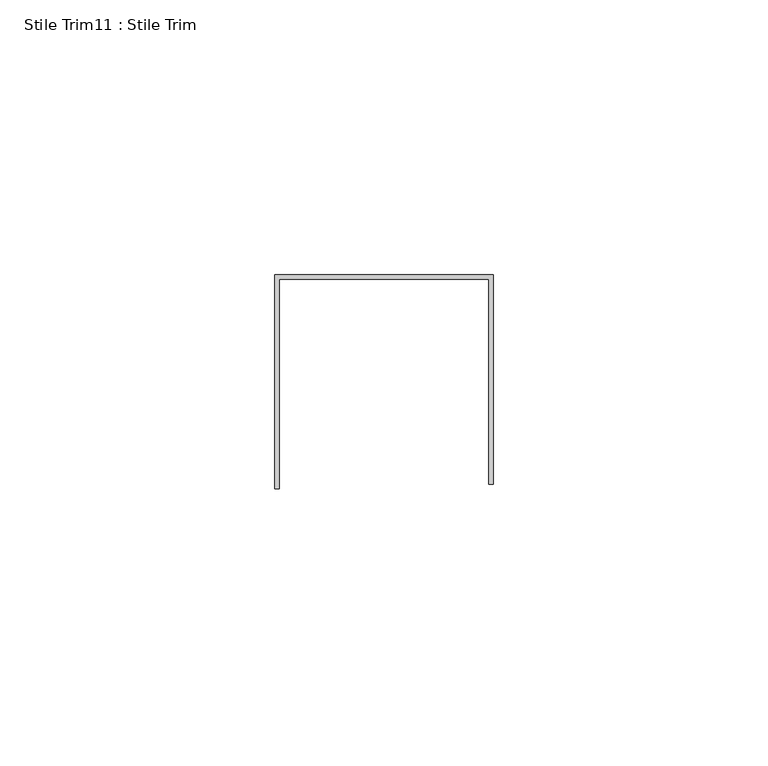
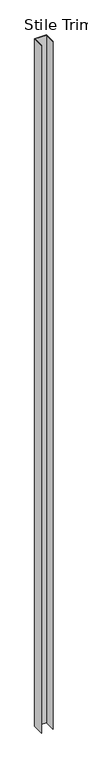
"""IFC4 building model written with IfcOpenShell, lengths in millimetres: proxy geometry, Stile Trim11 : Stile Trim."""

from ifc_helpers import new_model, si_unit, frame, origin, place, context, project, spatial, polyline, outline, extrude, source, transform, mapped, element, save


def stile_trim11_stile_trim_282884a6(model_context):
    return source(origin(), model_context, "Body", "SweptSolid", [
        extrude(outline(polyline([(587327.0060739, -536293.7663841), (587366.6808739, -536293.7663841), (587366.6808739, -536331.8663841), (587365.8934739, -536331.8663841), (587365.8934739, -536294.5537841), (587327.7934739, -536294.5537841), (587327.7934739, -536332.6537841), (587327.0060739, -536332.6537841), (587327.0060739, -536293.7663841)])), frame((0.0, 0.0, 12.7), z_axis=(0.0, 0.0, 1.0), x_axis=(1.0, 0.0, 0.0)), (0.0, 0.0, 1.0), 2425.7),
    ])


if __name__ == "__main__":
    model = new_model("IFC4")
    model_context = context("Model", 3, world=origin())
    ifc_project = project(units=[si_unit("LENGTHUNIT", "METRE", prefix="MILLI")], contexts=[model_context])
    site = spatial("IfcSite", under=ifc_project)
    building = spatial("IfcBuilding", under=site)
    placement = place(None, origin())
    stile_trim11_stile_trim_shape = stile_trim11_stile_trim_282884a6(model_context)
    element("IfcBuildingElementProxy", 1, Name="Stile Trim11 : Stile Trim", ObjectType="Stile Trim11 : Stile Trim", at=placement, inside=building, context=model_context, shape_type="MappedRepresentation", body=[
        mapped(stile_trim11_stile_trim_shape, transform((0.0, 0.0, 0.0), x_axis=(1.0, 0.0, 0.0), y_axis=(0.0, 1.0, 0.0), z_axis=(0.0, 0.0, 1.0))),
    ])
    save(model, "model.ifc")

# Revit data of these elements
# Element 1 (IfcBuildingElementProxy, "Stile Trim11 : Stile Trim")
#   Materials on its faces: "EDGE TRIM BY MTL PANEL MFR."
# Materials
#   "EDGE TRIM BY MTL PANEL MFR.": class "Generic", colour RGB 239 242 240, transparency 0, Cost = 0
